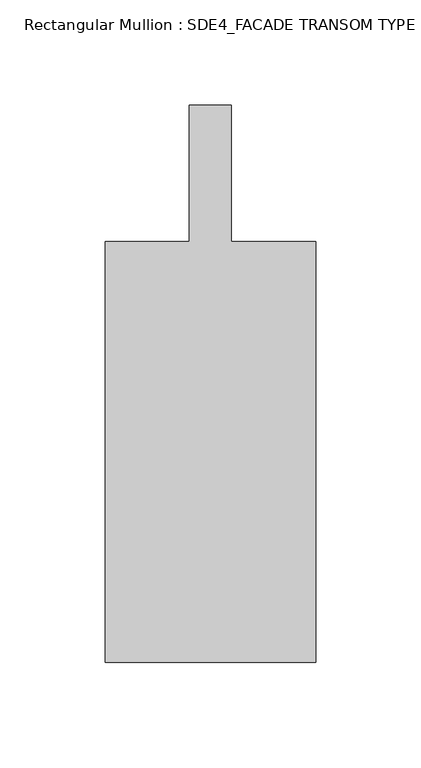
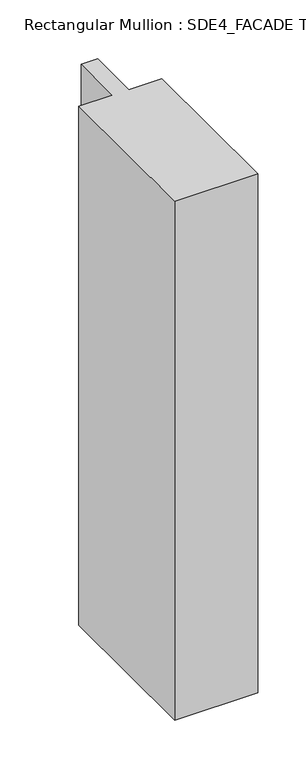
"""IFC4 building model written with IfcOpenShell, lengths in millimetres: member geometry, Rectangular Mullion : SDE4_FACADE TRANSOM TYPE 2."""

from ifc_helpers import new_model, si_unit, frame, origin, place, context, project, spatial, polyline, outline, extrude, source, transform, mapped, element, save


def rectangular_mullion_sde4_facade_transom_type_2_f51b2154(model_context):
    return source(origin(), model_context, "Body", "SweptSolid", [
        extrude(outline(polyline([(50.0, -132.5), (-50.0, -132.5), (-50.0, 67.5), (-10.0, 67.5), (-10.0, 132.5), (10.0, 132.5), (10.0, 67.5), (50.0, 67.5), (50.0, -132.5)])), frame((0.0, 0.0, -661.5000001), z_axis=(0.0, 0.0, 1.0), x_axis=(1.0, 0.0, 0.0)), (0.0, 0.0, 1.0), 661.5000001),
    ])


if __name__ == "__main__":
    model = new_model("IFC4")
    model_context = context("Model", 3, world=origin())
    ifc_project = project(units=[si_unit("LENGTHUNIT", "METRE", prefix="MILLI")], contexts=[model_context])
    site = spatial("IfcSite", under=ifc_project)
    building = spatial("IfcBuilding", under=site)
    placement = place(None, origin())
    rectangular_mullion_sde4_facade_transom_type_2_shape = rectangular_mullion_sde4_facade_transom_type_2_f51b2154(model_context)
    element("IfcMember", 1, ObjectType="Rectangular Mullion : SDE4_FACADE TRANSOM TYPE 2", at=placement, inside=building, context=model_context, shape_type="MappedRepresentation", body=[
        mapped(rectangular_mullion_sde4_facade_transom_type_2_shape, transform((0.0, 0.0, 0.0), x_axis=(1.0, 0.0, 0.0), y_axis=(0.0, 1.0, 0.0), z_axis=(0.0, 0.0, 1.0))),
    ])
    save(model, "model.ifc")

# Revit data of these elements
# Type "Rectangular Mullion : SDE4_FACADE TRANSOM TYPE 2"
#   built-in parameter 1007322 = 0.869423 (stored number, unit not read)
#   built-in parameter 1007321 = 0.164042 (stored number, unit not read)
#   built-in parameter 1007320 = 0.164042 (stored number, unit not read)
